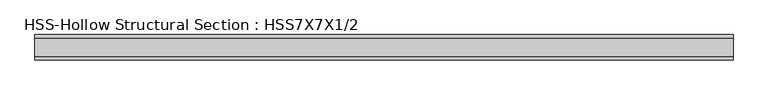
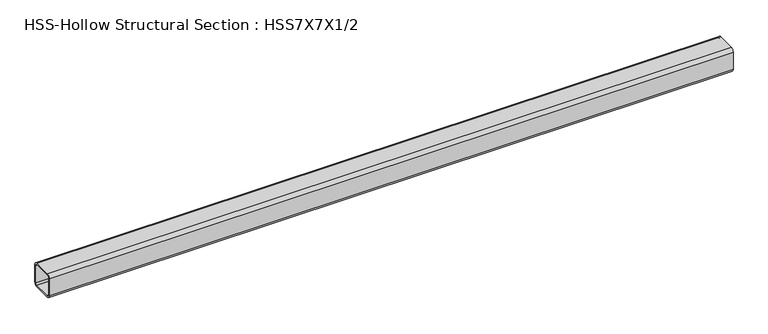
"""IFC4 building model written with IfcOpenShell, lengths in millimetres: member geometry, HSS-Hollow Structural Section : HSS7X7X1/2."""

from ifc_helpers import new_model, si_unit, point, frame, frame_2d, origin, place, context, project, spatial, polyline, circle_curve, trimmed, segment, composite_curve, outline, extrude, source, transform, mapped, element, save


def hss_hollow_structural_section_hss7x7x1_2_91102c0f(model_context):
    return source(origin(), model_context, "Body", "SweptSolid", [
        extrude(outline(composite_curve([segment(polyline([(88.9, 65.278), (88.9, -65.278)]), True, "CONTINUOUS"), segment(trimmed(circle_curve(frame_2d((65.278, -65.278)), 23.622), [point((88.9, -65.278))], [point((65.278, -88.9))], False, "CARTESIAN"), True, "CONTINUOUS"), segment(polyline([(65.278, -88.9), (-65.278, -88.9)]), True, "CONTINUOUS"), segment(trimmed(circle_curve(frame_2d((-65.278, -65.278)), 23.622), [point((-65.278, -88.9))], [point((-88.9, -65.278))], False, "CARTESIAN"), True, "CONTINUOUS"), segment(polyline([(-88.9, -65.278), (-88.9, 65.278)]), True, "CONTINUOUS"), segment(trimmed(circle_curve(frame_2d((-65.278, 65.278)), 23.622), [point((-88.9, 65.278))], [point((-65.278, 88.9))], False, "CARTESIAN"), True, "CONTINUOUS"), segment(polyline([(-65.278, 88.9), (65.278, 88.9)]), True, "CONTINUOUS"), segment(trimmed(circle_curve(frame_2d((65.278, 65.278)), 23.622), [point((65.278, 88.9))], [point((88.9, 65.278))], False, "CARTESIAN"), True, "CONTINUOUS")], self_intersect=False), holes=[composite_curve([segment(trimmed(circle_curve(frame_2d((-65.278, 65.278)), 11.811), [point((-65.278, 77.089))], [point((-77.089, 65.278))], True, "CARTESIAN"), True, "CONTINUOUS"), segment(polyline([(-77.089, 65.278), (-77.089, -65.278)]), True, "CONTINUOUS"), segment(trimmed(circle_curve(frame_2d((-65.278, -65.278)), 11.811), [point((-77.089, -65.278))], [point((-65.278, -77.089))], True, "CARTESIAN"), True, "CONTINUOUS"), segment(polyline([(-65.278, -77.089), (65.278, -77.089)]), True, "CONTINUOUS"), segment(trimmed(circle_curve(frame_2d((65.278, -65.278)), 11.811), [point((65.278, -77.089))], [point((77.089, -65.278))], True, "CARTESIAN"), True, "CONTINUOUS"), segment(polyline([(77.089, -65.278), (77.089, 65.278)]), True, "CONTINUOUS"), segment(trimmed(circle_curve(frame_2d((65.278, 65.278)), 11.811), [point((77.089, 65.278))], [point((65.278, 77.089))], True, "CARTESIAN"), True, "CONTINUOUS"), segment(polyline([(65.278, 77.089), (-65.278, 77.089)]), True, "CONTINUOUS")], self_intersect=False)]), frame((-2443.5496913, 0.0, 0.0), z_axis=(1.0, 0.0, 0.0), x_axis=(0.0, 1.0, 0.0)), (0.0, 0.0, 1.0), 4928.3274662),
    ])


if __name__ == "__main__":
    model = new_model("IFC4")
    model_context = context("Model", 3, world=origin())
    ifc_project = project(units=[si_unit("LENGTHUNIT", "METRE", prefix="MILLI")], contexts=[model_context])
    site = spatial("IfcSite", under=ifc_project)
    building = spatial("IfcBuilding", under=site)
    placement = place(None, origin())
    hss_hollow_structural_section_hss7x7x1_2_shape = hss_hollow_structural_section_hss7x7x1_2_91102c0f(model_context)
    element("IfcMember", 1, ObjectType="HSS-Hollow Structural Section : HSS7X7X1/2", at=placement, inside=building, context=model_context, shape_type="MappedRepresentation", body=[
        mapped(hss_hollow_structural_section_hss7x7x1_2_shape, transform((0.0, 0.0, 0.0), x_axis=(1.0, 0.0, 0.0), y_axis=(0.0, 1.0, 0.0), z_axis=(0.0, 0.0, 1.0))),
    ])
    save(model, "model.ifc")

# Revit data of these elements
# Type "HSS-Hollow Structural Section : HSS7X7X1/2"
#   Assembly Code = "B10"
#   Shape = "Square"
#   W = 41.9
#   Ht = 0' - 7"
#   Length [instance default] = 5' - 0"
#   b = 0' - 7"
#   kr = 0' - 0.93"
#   t = 0' - 0.465"
#   A = 0.0805556 SF
#   Structural Material [instance default] = Steel ASTM A500, Grade B, Rectangular and Square
# Element 1 (IfcMember, "HSS-Hollow Structural Section : HSS7X7X1/2")
#   Materials on its faces: "Steel ASTM A500, Grade B, Rectangular and Square"
# Materials
#   "Steel ASTM A500, Grade B, Rectangular and Square": class "Metal", colour RGB 199 199 199, transparency 0, Description = "Carbon steel", Cost = 0
